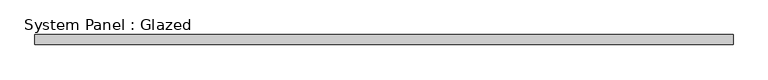
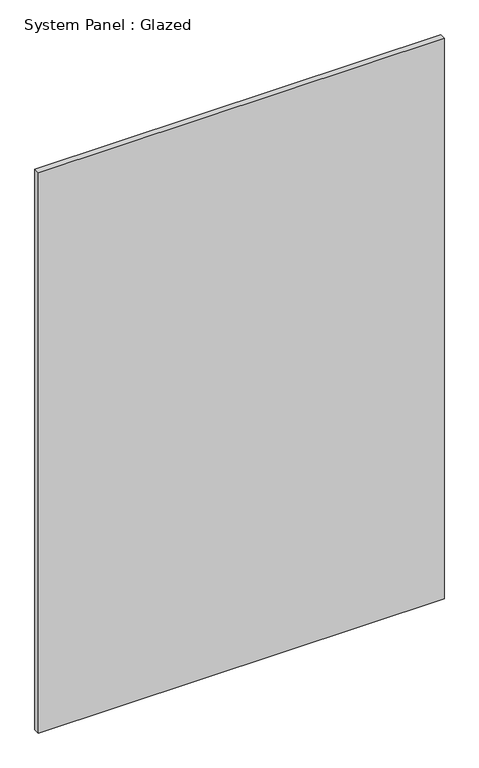
"""IFC4 building model written with IfcOpenShell, lengths in millimetres: plate geometry, System Panel : Glazed."""

from ifc_helpers import new_model, si_unit, origin, origin_with_axes, place, context, project, spatial, polyline, outline, extrude, source, transform, mapped, element, save


def system_panel_glazed_ae73c78b(model_context):
    return source(origin(), model_context, "Body", "SweptSolid", [
        extrude(outline(polyline([(882.65, 19.05), (-882.65, 19.05), (-882.65, 44.45), (882.65, 44.45), (882.65, 19.05)])), origin_with_axes(), (0.0, 0.0, 1.0), 2578.1),
    ])


if __name__ == "__main__":
    model = new_model("IFC4")
    model_context = context("Model", 3, world=origin())
    ifc_project = project(units=[si_unit("LENGTHUNIT", "METRE", prefix="MILLI")], contexts=[model_context])
    site = spatial("IfcSite", under=ifc_project)
    building = spatial("IfcBuilding", under=site)
    placement = place(None, origin())
    system_panel_glazed_shape = system_panel_glazed_ae73c78b(model_context)
    element("IfcPlate", 1, ObjectType="System Panel : Glazed", at=placement, inside=building, context=model_context, shape_type="MappedRepresentation", body=[
        mapped(system_panel_glazed_shape, transform((0.0, 0.0, 0.0), x_axis=(1.0, 0.0, 0.0), y_axis=(0.0, 1.0, 0.0), z_axis=(0.0, 0.0, 1.0))),
    ])
    save(model, "model.ifc")

# Revit data of these elements
# Type "System Panel : Glazed"
#   Construction Type Id = "GSP4R"
#   Analytic Construction = "1/8 in Pilkington single glazing"
#   Visual Light Transmittance = 0.9
#   Solar Heat Gain Coefficient = 0.86
#   Heat Transfer Coefficient (U) = 1.18115 BTU/(h·ft²·°F)
#   Define Thermal Properties by = 1
# Element 1 (IfcPlate, "System Panel : Glazed")
#   Materials on its faces: "Glass"
# Materials
#   "Glass": class "Glass", colour RGB 0 128 192, transparency 0.75, Description = "Soda Lime Glass", Cost = 0
